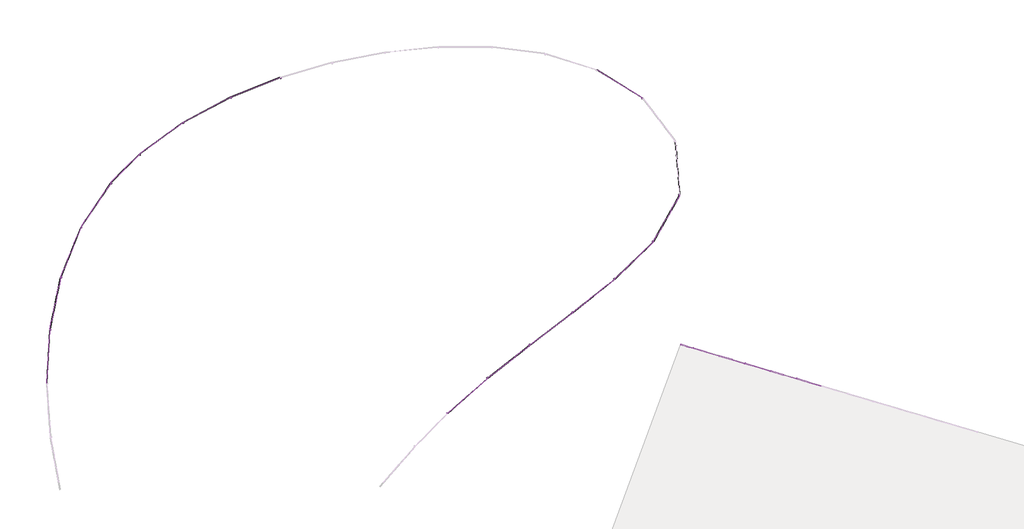
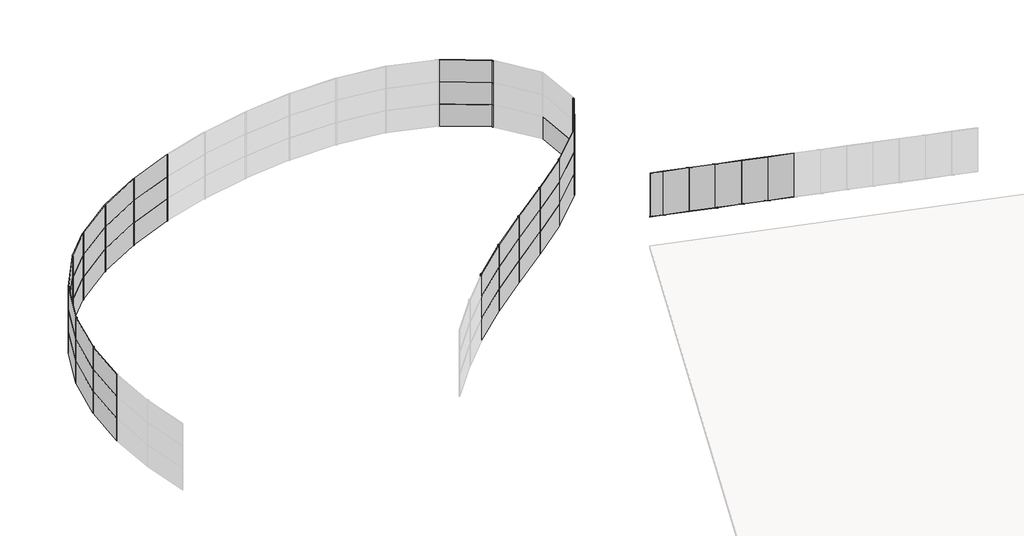
# One storey, part 4 of 5: 53 members, 52 plates.
"""IFC4 building model written with IfcOpenShell, lengths in millimetres."""

import ifcopenshell
import ifcopenshell.guid

model = None  # the IFC model being written
_history = None  # IfcOwnerHistory: only IFC2X3 demands one
_inside = {}  # id of a spatial element -> (the spatial element, [elements in it])
_under = {}  # id of a project, library or spatial element -> (it, [spatial elements below it])
_declared = {}  # id of a project -> (the project, [libraries it declares])
_typed = {}  # id of a type object -> (the type object, [elements of that type])
_made_of = {}  # id of a material, layer set ... -> (it, [elements and type objects made of it])


def new_model(schema):
    """Start an empty IFC model of exactly this schema.

    Asked for "IFC4X3", IfcOpenShell would pick the latest addendum, in which some entities
    have other attributes; the version numbers below select the first issue.
    IFC2X3 requires an IfcOwnerHistory on every rooted entity: one is made here for all.
    """
    global model, _history
    if schema == "IFC4X3":
        model = ifcopenshell.file(schema_version=(4, 3, 0, 0))
    else:
        model = ifcopenshell.file(schema=schema)
    _inside.clear()
    _under.clear()
    _declared.clear()
    _typed.clear()
    _made_of.clear()
    _history = None
    if model.schema == "IFC2X3":
        org = make("IfcOrganization", Name="unknown")
        user = make(
            "IfcPersonAndOrganization",
            ThePerson=make("IfcPerson", FamilyName="unknown"),
            TheOrganization=org,
        )
        app = make(
            "IfcApplication",
            ApplicationDeveloper=org,
            Version="unknown",
            ApplicationFullName="unknown",
            ApplicationIdentifier="unknown",
        )
        _history = make(
            "IfcOwnerHistory",
            OwningUser=user,
            OwningApplication=app,
            ChangeAction="ADDED",
            CreationDate=0,
        )
    return model


def make(cls, **values):
    """One entity of the class cls with the attributes given. An attribute that is None is left unset."""
    return model.create_entity(
        cls, **{name: value for name, value in values.items() if value is not None}
    )


def rooted(cls, **values):
    """An entity with a GlobalId (a new one), such as an element, a storey or a relation."""
    return make(cls, GlobalId=ifcopenshell.guid.new(), OwnerHistory=_history, **values)


def si_unit(unit_type, name, prefix=None):
    """IfcSIUnit, for example si_unit("LENGTHUNIT", "METRE", prefix="MILLI")."""
    return make("IfcSIUnit", UnitType=unit_type, Prefix=prefix, Name=name)


def assignment(units):
    """IfcUnitAssignment: the units of a project."""
    return None if units is None else make("IfcUnitAssignment", Units=units)


def point(xyz):
    """IfcCartesianPoint."""
    return None if xyz is None else make("IfcCartesianPoint", Coordinates=xyz)


def direction(xyz):
    """IfcDirection."""
    return None if xyz is None else make("IfcDirection", DirectionRatios=xyz)


def frame(location, z_axis=None, x_axis=None):
    """IfcAxis2Placement3D, a coordinate frame: its origin and axes. An axis left out is left unset."""
    return make(
        "IfcAxis2Placement3D",
        Location=point(location),
        Axis=direction(z_axis),
        RefDirection=direction(x_axis),
    )


def frame_2d(location, x_axis=None):
    """IfcAxis2Placement2D, a coordinate frame in the plane: its origin and x axis."""
    return make(
        "IfcAxis2Placement2D", Location=point(location), RefDirection=direction(x_axis)
    )


def origin():
    """The frame at (0, 0, 0) with its axes left unset."""
    return frame((0.0, 0.0, 0.0))


def origin_with_axes():
    """The frame at (0, 0, 0) with the z axis (0, 0, 1) and the x axis (1, 0, 0) written out."""
    return frame((0.0, 0.0, 0.0), z_axis=(0.0, 0.0, 1.0), x_axis=(1.0, 0.0, 0.0))


def origin_2d():
    """The frame at (0, 0) in the plane with its x axis left unset."""
    return frame_2d((0.0, 0.0))


def place(relative_to, where):
    """IfcLocalPlacement: puts the frame where relative to a parent placement (None: the world)."""
    return make(
        "IfcLocalPlacement", PlacementRelTo=relative_to, RelativePlacement=where
    )


def context(
    kind, dimensions, precision=None, world=None, true_north=None, identifier=None
):
    """IfcGeometricRepresentationContext, for example the 3D "Model" context."""
    return make(
        "IfcGeometricRepresentationContext",
        ContextIdentifier=identifier,
        ContextType=kind,
        CoordinateSpaceDimension=dimensions,
        Precision=precision,
        WorldCoordinateSystem=world,
        TrueNorth=true_north,
    )


def project(units=None, contexts=None):
    """IfcProject with its units and contexts."""
    return rooted(
        "IfcProject",
        Name="project",
        RepresentationContexts=contexts,
        UnitsInContext=assignment(units),
    )


def spatial(cls, under=None, at=None, **own):
    """A site, building, storey or space (cls), placed at a placement, below another one or the project."""
    s = rooted(cls, ObjectPlacement=at, **own)
    if under is not None:
        _under.setdefault(under.id(), (under, []))[1].append(s)
    return s


def polyline(points):
    """IfcPolyline through the points."""
    return make("IfcPolyline", Points=[point(p) for p in points])


def circle_curve(where, radius):
    """IfcCircle in the frame where."""
    return make("IfcCircle", Position=where, Radius=radius)


def trimmed(basis, trim1, trim2, sense, master):
    """IfcTrimmedCurve: the piece of a basis curve between two trims."""
    return make(
        "IfcTrimmedCurve",
        BasisCurve=basis,
        Trim1=trim1,
        Trim2=trim2,
        SenseAgreement=sense,
        MasterRepresentation=master,
    )


def segment(curve, same_sense, transition):
    """IfcCompositeCurveSegment."""
    return make(
        "IfcCompositeCurveSegment",
        Transition=transition,
        SameSense=same_sense,
        ParentCurve=curve,
    )


def composite_curve(segments, self_intersect=None):
    """IfcCompositeCurve: segments joined end to end."""
    return make("IfcCompositeCurve", Segments=segments, SelfIntersect=self_intersect)


def outline(outer, holes=None, kind="AREA"):
    """IfcArbitraryClosedProfileDef: a profile drawn as a closed curve; with holes, ...WithVoids."""
    if holes is None:
        return make("IfcArbitraryClosedProfileDef", ProfileType=kind, OuterCurve=outer)
    return make(
        "IfcArbitraryProfileDefWithVoids",
        ProfileType=kind,
        OuterCurve=outer,
        InnerCurves=holes,
    )


def extrude(swept, where, along, depth):
    """IfcExtrudedAreaSolid: the profile swept, set in the frame where, extruded along a direction by depth."""
    return make(
        "IfcExtrudedAreaSolid",
        SweptArea=swept,
        Position=where,
        ExtrudedDirection=direction(along),
        Depth=depth,
    )


def shape(context_of_items, identifier, shape_type, items):
    """IfcShapeRepresentation: the items that make up one representation, for example the "Body"."""
    return make(
        "IfcShapeRepresentation",
        ContextOfItems=context_of_items,
        RepresentationIdentifier=identifier,
        RepresentationType=shape_type,
        Items=items,
    )


def source(mapping_origin, context_of_items, identifier, shape_type, items):
    """IfcRepresentationMap: a shape defined once, which mapped items show again and again."""
    return make(
        "IfcRepresentationMap",
        MappingOrigin=mapping_origin,
        MappedRepresentation=shape(context_of_items, identifier, shape_type, items),
    )


def transform(
    local_origin,
    x_axis=None,
    y_axis=None,
    z_axis=None,
    scale=None,
    scale2=None,
    scale3=None,
    uniform=True,
):
    """IfcCartesianTransformationOperator3D, or its non-uniform kind. x_axis, y_axis, z_axis: its Axis1, 2, 3."""
    if uniform:
        return make(
            "IfcCartesianTransformationOperator3D",
            Axis1=direction(x_axis),
            Axis2=direction(y_axis),
            LocalOrigin=point(local_origin),
            Scale=scale,
            Axis3=direction(z_axis),
        )
    return make(
        "IfcCartesianTransformationOperator3DnonUniform",
        Axis1=direction(x_axis),
        Axis2=direction(y_axis),
        LocalOrigin=point(local_origin),
        Scale=scale,
        Axis3=direction(z_axis),
        Scale2=scale2,
        Scale3=scale3,
    )


def mapped(mapping_source, mapping_target):
    """IfcMappedItem: shows the shape of a source again, moved by a transform."""
    return make(
        "IfcMappedItem", MappingSource=mapping_source, MappingTarget=mapping_target
    )


def made_of(thing, what):
    """Note that an element or type object is made of a material, layer set ...; save() writes the relation."""
    if what is not None:
        _made_of.setdefault(what.id(), (what, []))[1].append(thing)
    return thing


def element(
    cls,
    number,
    at=None,
    inside=None,
    cuts=None,
    type_object=None,
    material=None,
    context=None,
    identifier="Body",
    shape_type=None,
    held_by="IfcProductDefinitionShape",
    body=None,
    shapes=None,
    **own,
):
    """One element of the class cls, such as IfcWall. Its Tag is "e" and its number.

    at: its placement. inside: the storey or other place that contains it. cuts: it is an
    opening in that element (IfcRelVoidsElement). A single representation is given by context,
    identifier, shape_type and body (its items); several are given by shapes. held_by: the class
    of the entity that holds the representations. save() writes the other relations.
    """
    e = rooted(cls, Tag="e%d" % number, ObjectPlacement=at, **own)
    if body is not None:
        shapes = [shape(context, identifier, shape_type, body)]
    if shapes is not None:
        e.Representation = make(held_by, Representations=shapes)
    if inside is not None:
        _inside.setdefault(inside.id(), (inside, []))[1].append(e)
    if cuts is not None:
        rooted(
            "IfcRelVoidsElement", RelatingBuildingElement=cuts, RelatedOpeningElement=e
        )
    if type_object is not None:
        _typed.setdefault(type_object.id(), (type_object, []))[1].append(e)
    return made_of(e, material)


def aggregate(whole, parts):
    """IfcRelAggregates: a whole, such as a stair, and the parts it consists of."""
    return rooted("IfcRelAggregates", RelatingObject=whole, RelatedObjects=parts)


def save(model, path):
    """Write the relations noted so far, then the file.

    IfcRelAggregates (storeys below a building ...), IfcRelContainedInSpatialStructure (elements
    in a storey), IfcRelDefinesByType, IfcRelAssociatesMaterial and IfcRelDeclares: one each for
    every whole, place, type object, material and project.
    """
    for whole, parts in _under.values():
        aggregate(whole, parts)
    for where, things in _inside.values():
        rooted(
            "IfcRelContainedInSpatialStructure",
            RelatedElements=things,
            RelatingStructure=where,
        )
    for kind, things in _typed.values():
        rooted("IfcRelDefinesByType", RelatedObjects=things, RelatingType=kind)
    for what, things in _made_of.values():
        rooted("IfcRelAssociatesMaterial", RelatedObjects=things, RelatingMaterial=what)
    for by, libraries in _declared.values():
        rooted("IfcRelDeclares", RelatingContext=by, RelatedDefinitions=libraries)
    model.write(path)


def montante_circular_25_mm_raio_36e581cf(model_context):
    return source(origin(), model_context, "Body", "SweptSolid", [
        extrude(outline(composite_curve([segment(trimmed(circle_curve(origin_2d(), 25.0), [point((25.0, 0.0))], [point((-25.0, 0.0))], False, "CARTESIAN"), True, "CONTINUOUS"), segment(trimmed(circle_curve(origin_2d(), 25.0), [point((-25.0, 0.0))], [point((25.0, 0.0))], False, "CARTESIAN"), True, "CONTINUOUS")], self_intersect=False)), frame((0.0, 0.0, -1500.0), z_axis=(0.0, 0.0, 1.0), x_axis=(1.0, 0.0, 0.0)), (0.0, 0.0, 1.0), 1500.0),
    ])


def montante_circular_25_mm_raio_a1f35a82(model_context):
    return source(origin(), model_context, "Body", "SweptSolid", [
        extrude(outline(composite_curve([segment(trimmed(circle_curve(origin_2d(), 25.0), [point((25.0, 0.0))], [point((-25.0, 0.0))], False, "CARTESIAN"), True, "CONTINUOUS"), segment(trimmed(circle_curve(origin_2d(), 25.0), [point((-25.0, 0.0))], [point((25.0, 0.0))], False, "CARTESIAN"), True, "CONTINUOUS")], self_intersect=False)), frame((0.0, 0.0, -727.4383788), z_axis=(0.0, 0.0, 1.0), x_axis=(1.0, 0.0, 0.0)), (0.0, 0.0, 1.0), 727.4383788),
    ])


def montante_circular_25_mm_raio_ce826986(model_context):
    return source(origin(), model_context, "Body", "SweptSolid", [
        extrude(outline(composite_curve([segment(trimmed(circle_curve(frame_2d((-25.0, 0.0)), 25.0), [point((0.0, 0.0))], [point((-50.0, 0.0))], False, "CARTESIAN"), True, "CONTINUOUS"), segment(trimmed(circle_curve(frame_2d((-25.0, 0.0)), 25.0), [point((-50.0, 0.0))], [point((0.0, 0.0))], False, "CARTESIAN"), True, "CONTINUOUS")], self_intersect=False)), frame((0.0, 0.0, -1500.0), z_axis=(0.0, 0.0, 1.0), x_axis=(1.0, 0.0, 0.0)), (0.0, 0.0, 1.0), 1500.0),
    ])


def painel_do_sistema_5ef9eced(model_context):
    return source(origin(), model_context, "Body", "SweptSolid", [
        extrude(outline(polyline([(1475.0, 24.5), (-1475.0, 24.5), (-1475.0, 49.5), (1475.0, 49.5), (1475.0, 24.5)])), origin_with_axes(), (0.0, 0.0, 1.0), 1500.0),
    ])


def painel_do_sistema_bf426e09(model_context):
    return source(origin(), model_context, "Body", "SweptSolid", [
        extrude(outline(polyline([(1475.0, 24.5), (-1475.0, 24.5), (-1475.0, 49.5), (1475.0, 49.5), (1475.0, 24.5)])), origin_with_axes(), (0.0, 0.0, 1.0), 727.4383788),
    ])


def painel_do_sistema_619734db(model_context):
    return source(origin(), model_context, "Body", "SweptSolid", [
        extrude(outline(polyline([(1462.5000305, -49.5), (-1462.5000305, -49.5), (-1462.5000305, -24.5), (1462.5000305, -24.5), (1462.5000305, -49.5)])), origin_with_axes(), (0.0, 0.0, 1.0), 1500.0),
    ])


def painel_do_sistema_9c2734b9(model_context):
    return source(origin(), model_context, "Body", "SweptSolid", [
        extrude(outline(polyline([(1462.5000336, -49.5), (-1462.5000336, -49.5), (-1462.5000336, -24.5), (1462.5000336, -24.5), (1462.5000336, -49.5)])), origin_with_axes(), (0.0, 0.0, 1.0), 1500.0),
    ])


def painel_do_sistema_85ccde5d(model_context):
    return source(origin(), model_context, "Body", "SweptSolid", [
        extrude(outline(polyline([(1475.0, -49.5), (-1475.0, -49.5), (-1475.0, -24.5), (1475.0, -24.5), (1475.0, -49.5)])), origin_with_axes(), (0.0, 0.0, 1.0), 1500.0),
    ])


def painel_do_sistema_91df381f(model_context):
    return source(origin(), model_context, "Body", "SweptSolid", [
        extrude(outline(polyline([(1110.3819696, -49.5), (-1110.3819696, -49.5), (-1110.3819696, -24.5), (1110.3819696, -24.5), (1110.3819696, -49.5)])), origin_with_axes(), (0.0, 0.0, 1.0), 1500.0),
    ])


model = new_model("IFC4")

# Units and contexts
model_context = context("Model", 3, world=origin())
ifc_project = project(units=[si_unit("LENGTHUNIT", "METRE", prefix="MILLI")], contexts=[model_context])

# Site, building, storey
site = spatial("IfcSite", under=ifc_project)
building = spatial("IfcBuilding", under=site)
storey = spatial("IfcBuildingStorey", under=building, Name="Nível 2", Elevation=4000.0)

# Members
placement = place(None, origin())
montante_circular_25_mm_raio_shape = montante_circular_25_mm_raio_36e581cf(model_context)
element("IfcMember", 1, ObjectType="Montante circular : 25 mm Raio", at=placement, inside=storey, context=model_context, shape_type="MappedRepresentation", body=[
    mapped(montante_circular_25_mm_raio_shape, transform((-73.9726554, 31091.8210426, 6000.000015), x_axis=(0.0, 0.0, 1.0), y_axis=(0.28318378939534855, 0.9590656606425293, 0.0), z_axis=(-0.9590656606425293, 0.28318378939534855, 0.0))),
])
element("IfcMember", 2, ObjectType="Montante circular : 25 mm Raio", at=placement, inside=storey, context=model_context, shape_type="MappedRepresentation", body=[
    mapped(montante_circular_25_mm_raio_shape, transform((-1512.5711463, 31516.5967267, 6000.000015), x_axis=(0.0, 0.0, 1.0), y_axis=(0.28318378939534644, 0.9590656606425298, 0.0), z_axis=(-0.9590656606425298, 0.28318378939534644, 0.0))),
])
element("IfcMember", 3, ObjectType="Montante circular : 25 mm Raio", at=placement, inside=storey, context=model_context, shape_type="MappedRepresentation", body=[
    mapped(montante_circular_25_mm_raio_shape, transform((-2951.1696373, 31941.3724108, 6000.000015), x_axis=(0.0, 0.0, 1.0), y_axis=(0.2831837893953519, 0.9590656606425282, 0.0), z_axis=(-0.9590656606425281, 0.2831837893953518, 0.0))),
])
element("IfcMember", 4, ObjectType="Montante circular : 25 mm Raio", at=placement, inside=storey, context=model_context, shape_type="MappedRepresentation", body=[
    mapped(montante_circular_25_mm_raio_shape, transform((-4389.7681283, 32366.1480949, 6000.000015), x_axis=(0.0, 0.0, 1.0), y_axis=(0.28318378939534594, 0.95906566064253, 0.0), z_axis=(-0.95906566064253, 0.28318378939534594, 0.0))),
])
element("IfcMember", 5, ObjectType="Montante circular : 25 mm Raio", at=placement, inside=storey, context=model_context, shape_type="MappedRepresentation", body=[
    mapped(montante_circular_25_mm_raio_shape, transform((-5828.3666192, 32790.923779, 6000.000015), x_axis=(0.0, 0.0, 1.0), y_axis=(0.283183789395347, 0.9590656606425296, 0.0), z_axis=(-0.9590656606425296, 0.283183789395347, 0.0))),
])
element("IfcMember", 6, ObjectType="Montante circular : 25 mm Raio", at=placement, inside=storey, context=model_context, shape_type="MappedRepresentation", body=[
    mapped(montante_circular_25_mm_raio_shape, transform((-40020.7762885, 39520.8946952, 4500.0), x_axis=(-0.4655884926939391, -0.8850013307735677, 0.0), y_axis=(-0.8850013307735677, 0.4655884926939391, 0.0), z_axis=(0.0, 0.0, -1.0))),
])
element("IfcMember", 7, ObjectType="Montante circular : 25 mm Raio", at=placement, inside=storey, context=model_context, shape_type="MappedRepresentation", body=[
    mapped(montante_circular_25_mm_raio_shape, transform((-41145.2595981, 36739.6113068, 4500.0), x_axis=(-0.28540905537136674, -0.958405796681147, 0.0), y_axis=(-0.958405796681147, 0.28540905537136674, 0.0), z_axis=(0.0, 0.0, -1.0))),
])
element("IfcMember", 8, ObjectType="Montante circular : 25 mm Raio", at=placement, inside=storey, context=model_context, shape_type="MappedRepresentation", body=[
    mapped(montante_circular_25_mm_raio_shape, transform((-41757.3897475, 33802.725766, 4500.0), x_axis=(-0.12631233821712995, -0.9919905207279561, 0.0), y_axis=(-0.9919905207279561, 0.12631233821712995, 0.0), z_axis=(0.0, 0.0, -1.0))),
])
element("IfcMember", 9, ObjectType="Montante circular : 25 mm Raio", at=placement, inside=storey, context=model_context, shape_type="MappedRepresentation", body=[
    mapped(montante_circular_25_mm_raio_shape, transform((-40020.7762885, 39520.8946952, 6000.0), x_axis=(-0.46558849269393926, -0.8850013307735677, 0.0), y_axis=(-0.8850013307735677, 0.46558849269393926, 0.0), z_axis=(0.0, 0.0, -1.0))),
])
element("IfcMember", 10, ObjectType="Montante circular : 25 mm Raio", at=placement, inside=storey, context=model_context, shape_type="MappedRepresentation", body=[
    mapped(montante_circular_25_mm_raio_shape, transform((-41145.2595981, 36739.6113068, 6000.0), x_axis=(-0.2854090553713671, -0.9584057966811469, 0.0), y_axis=(-0.9584057966811469, 0.2854090553713671, 0.0), z_axis=(0.0, 0.0, -1.0))),
])
element("IfcMember", 11, ObjectType="Montante circular : 25 mm Raio", at=placement, inside=storey, context=model_context, shape_type="MappedRepresentation", body=[
    mapped(montante_circular_25_mm_raio_shape, transform((-41757.3897475, 33802.725766, 6000.0), x_axis=(-0.12631233821712953, -0.9919905207279561, 0.0), y_axis=(-0.9919905207279561, 0.12631233821712953, 0.0), z_axis=(0.0, 0.0, -1.0))),
])
element("IfcMember", 12, ObjectType="Montante circular : 25 mm Raio", at=placement, inside=storey, context=model_context, shape_type="MappedRepresentation", body=[
    mapped(montante_circular_25_mm_raio_shape, transform((-40020.7762885, 39520.8946952, 7500.0), x_axis=(-0.4655884926939391, -0.8850013307735677, 0.0), y_axis=(-0.8850013307735677, 0.4655884926939391, 0.0), z_axis=(0.0, 0.0, -1.0))),
])
element("IfcMember", 13, ObjectType="Montante circular : 25 mm Raio", at=placement, inside=storey, context=model_context, shape_type="MappedRepresentation", body=[
    mapped(montante_circular_25_mm_raio_shape, transform((-41145.2595981, 36739.6113068, 7500.0), x_axis=(-0.28540905537136674, -0.958405796681147, 0.0), y_axis=(-0.958405796681147, 0.28540905537136674, 0.0), z_axis=(0.0, 0.0, -1.0))),
])
element("IfcMember", 14, ObjectType="Montante circular : 25 mm Raio", at=placement, inside=storey, context=model_context, shape_type="MappedRepresentation", body=[
    mapped(montante_circular_25_mm_raio_shape, transform((-41757.3897475, 33802.725766, 7500.0), x_axis=(-0.12631233821712995, -0.9919905207279561, 0.0), y_axis=(-0.9919905207279561, 0.12631233821712995, 0.0), z_axis=(0.0, 0.0, -1.0))),
])
element("IfcMember", 15, ObjectType="Montante circular : 25 mm Raio", at=placement, inside=storey, context=model_context, shape_type="MappedRepresentation", body=[
    mapped(montante_circular_25_mm_raio_shape, transform((-17353.3233761, 31118.8559936, 4500.0), x_axis=(0.7724767966577648, 0.6350429895883886, 0.0), y_axis=(0.6350429895883886, -0.7724767966577648, 0.0), z_axis=(0.0, 0.0, -1.0))),
])
element("IfcMember", 16, ObjectType="Montante circular : 25 mm Raio", at=placement, inside=storey, context=model_context, shape_type="MappedRepresentation", body=[
    mapped(montante_circular_25_mm_raio_shape, transform((-14996.1891623, 32974.6356945, 4500.0), x_axis=(0.7952150611070873, 0.6063274747102028, 0.0), y_axis=(0.6063274747102028, -0.7952150611070873, 0.0), z_axis=(0.0, 0.0, -1.0))),
])
element("IfcMember", 17, ObjectType="Montante circular : 25 mm Raio", at=placement, inside=storey, context=model_context, shape_type="MappedRepresentation", body=[
    mapped(montante_circular_25_mm_raio_shape, transform((-12604.1298635, 34785.1749266, 4500.0), x_axis=(0.7953870623365296, 0.6061018240095187, 0.0), y_axis=(0.6061018240095187, -0.7953870623365296, 0.0), z_axis=(0.0, 0.0, -1.0))),
])
element("IfcMember", 18, ObjectType="Montante circular : 25 mm Raio", at=placement, inside=storey, context=model_context, shape_type="MappedRepresentation", body=[
    mapped(montante_circular_25_mm_raio_shape, transform((-10255.474771, 36651.6741247, 4500.0), x_axis=(0.7627263023971693, 0.6467214142361005, 0.0), y_axis=(0.6467214142361005, -0.7627263023971693, 0.0), z_axis=(0.0, 0.0, -1.0))),
])
element("IfcMember", 19, ObjectType="Montante circular : 25 mm Raio", at=placement, inside=storey, context=model_context, shape_type="MappedRepresentation", body=[
    mapped(montante_circular_25_mm_raio_shape, transform((-8101.871437, 38740.2125323, 4500.0), x_axis=(0.6490334571140042, 0.7607598645739956, 0.0), y_axis=(0.7607598645739956, -0.6490334571140042, 0.0), z_axis=(0.0, 0.0, -1.0))),
])
element("IfcMember", 20, ObjectType="Montante circular : 25 mm Raio", at=placement, inside=storey, context=model_context, shape_type="MappedRepresentation", body=[
    mapped(montante_circular_25_mm_raio_shape, transform((-6627.5874319, 41352.9671461, 4500.0), x_axis=(0.24827563424230142, 0.9686894287859154, 0.0), y_axis=(0.9686894287859154, -0.24827563424230142, 0.0), z_axis=(0.0, 0.0, -1.0))),
])
element("IfcMember", 21, ObjectType="Montante circular : 25 mm Raio", at=placement, inside=storey, context=model_context, shape_type="MappedRepresentation", body=[
    mapped(montante_circular_25_mm_raio_shape, transform((-8685.5307871, 46730.4667655, 4500.0), x_axis=(-0.7608105002607386, 0.6489741001711892, 0.0), y_axis=(0.6489741001711892, 0.7608105002607386, 0.0), z_axis=(0.0, 0.0, -1.0))),
])
element("IfcMember", 22, ObjectType="Montante circular : 25 mm Raio", at=placement, inside=storey, context=model_context, shape_type="MappedRepresentation", body=[
    mapped(montante_circular_25_mm_raio_shape, transform((-28892.5410808, 47874.3709699, 4500.0), x_axis=(-0.9471529213375351, -0.3207823929111028, 0.0), y_axis=(-0.3207823929111028, 0.9471529213375351, 0.0), z_axis=(0.0, 0.0, -1.0))),
])
element("IfcMember", 23, ObjectType="Montante circular : 25 mm Raio", at=placement, inside=storey, context=model_context, shape_type="MappedRepresentation", body=[
    mapped(montante_circular_25_mm_raio_shape, transform((-31682.4252949, 46771.3994961, 4500.0), x_axis=(-0.9093535544571358, -0.41602417357188853, 0.0), y_axis=(-0.41602417357188853, 0.9093535544571358, 0.0), z_axis=(0.0, 0.0, -1.0))),
])
element("IfcMember", 24, ObjectType="Montante circular : 25 mm Raio", at=placement, inside=storey, context=model_context, shape_type="MappedRepresentation", body=[
    mapped(montante_circular_25_mm_raio_shape, transform((-34331.1697585, 45362.7999198, 4500.0), x_axis=(-0.850927589483555, -0.5252830070121312, 0.0), y_axis=(-0.5252830070121312, 0.850927589483555, 0.0), z_axis=(0.0, 0.0, -1.0))),
])
element("IfcMember", 25, ObjectType="Montante circular : 25 mm Raio", at=placement, inside=storey, context=model_context, shape_type="MappedRepresentation", body=[
    mapped(montante_circular_25_mm_raio_shape, transform((-36756.8303499, 43597.5320378, 4500.0), x_axis=(-0.7567414762597636, -0.6537142633507346, 0.0), y_axis=(-0.6537142633507346, 0.7567414762597636, 0.0), z_axis=(0.0, 0.0, -1.0))),
])
element("IfcMember", 26, ObjectType="Montante circular : 25 mm Raio", at=placement, inside=storey, context=model_context, shape_type="MappedRepresentation", body=[
    mapped(montante_circular_25_mm_raio_shape, transform((-17353.3233761, 31118.8559936, 6000.0), x_axis=(0.7724767966577647, 0.6350429895883888, 0.0), y_axis=(0.6350429895883888, -0.7724767966577647, 0.0), z_axis=(0.0, 0.0, -1.0))),
])
element("IfcMember", 27, ObjectType="Montante circular : 25 mm Raio", at=placement, inside=storey, context=model_context, shape_type="MappedRepresentation", body=[
    mapped(montante_circular_25_mm_raio_shape, transform((-14996.1891623, 32974.6356945, 6000.0), x_axis=(0.7952150611070872, 0.6063274747102029, 0.0), y_axis=(0.6063274747102029, -0.7952150611070872, 0.0), z_axis=(0.0, 0.0, -1.0))),
])
element("IfcMember", 28, ObjectType="Montante circular : 25 mm Raio", at=placement, inside=storey, context=model_context, shape_type="MappedRepresentation", body=[
    mapped(montante_circular_25_mm_raio_shape, transform((-12604.1298635, 34785.1749266, 6000.0), x_axis=(0.7953870623365296, 0.6061018240095187, 0.0), y_axis=(0.6061018240095187, -0.7953870623365296, 0.0), z_axis=(0.0, 0.0, -1.0))),
])
element("IfcMember", 29, ObjectType="Montante circular : 25 mm Raio", at=placement, inside=storey, context=model_context, shape_type="MappedRepresentation", body=[
    mapped(montante_circular_25_mm_raio_shape, transform((-10255.474771, 36651.6741247, 6000.0), x_axis=(0.7627263023971692, 0.6467214142361007, 0.0), y_axis=(0.6467214142361007, -0.7627263023971692, 0.0), z_axis=(0.0, 0.0, -1.0))),
])
element("IfcMember", 30, ObjectType="Montante circular : 25 mm Raio", at=placement, inside=storey, context=model_context, shape_type="MappedRepresentation", body=[
    mapped(montante_circular_25_mm_raio_shape, transform((-8101.871437, 38740.2125323, 6000.0), x_axis=(0.6490334571140043, 0.7607598645739955, 0.0), y_axis=(0.7607598645739955, -0.6490334571140043, 0.0), z_axis=(0.0, 0.0, -1.0))),
])
element("IfcMember", 31, ObjectType="Montante circular : 25 mm Raio", at=placement, inside=storey, context=model_context, shape_type="MappedRepresentation", body=[
    mapped(montante_circular_25_mm_raio_shape, transform((-6627.5874319, 41352.9671461, 6000.0), x_axis=(0.24827563424230267, 0.968689428785915, 0.0), y_axis=(0.968689428785915, -0.24827563424230267, 0.0), z_axis=(0.0, 0.0, -1.0))),
])
element("IfcMember", 32, ObjectType="Montante circular : 25 mm Raio", at=placement, inside=storey, context=model_context, shape_type="MappedRepresentation", body=[
    mapped(montante_circular_25_mm_raio_shape, transform((-8685.5307871, 46730.4667655, 6000.0), x_axis=(-0.7608105002607383, 0.6489741001711896, 0.0), y_axis=(0.6489741001711896, 0.7608105002607383, 0.0), z_axis=(0.0, 0.0, -1.0))),
])
element("IfcMember", 33, ObjectType="Montante circular : 25 mm Raio", at=placement, inside=storey, context=model_context, shape_type="MappedRepresentation", body=[
    mapped(montante_circular_25_mm_raio_shape, transform((-28892.5410808, 47874.3709699, 6000.0), x_axis=(-0.9471529213375351, -0.32078239291110255, 0.0), y_axis=(-0.32078239291110255, 0.9471529213375351, 0.0), z_axis=(0.0, 0.0, -1.0))),
])
element("IfcMember", 34, ObjectType="Montante circular : 25 mm Raio", at=placement, inside=storey, context=model_context, shape_type="MappedRepresentation", body=[
    mapped(montante_circular_25_mm_raio_shape, transform((-31682.4252949, 46771.3994961, 6000.0), x_axis=(-0.9093535544571357, -0.4160241735718888, 0.0), y_axis=(-0.4160241735718888, 0.9093535544571357, 0.0), z_axis=(0.0, 0.0, -1.0))),
])
element("IfcMember", 35, ObjectType="Montante circular : 25 mm Raio", at=placement, inside=storey, context=model_context, shape_type="MappedRepresentation", body=[
    mapped(montante_circular_25_mm_raio_shape, transform((-34331.1697585, 45362.7999198, 6000.0), x_axis=(-0.850927589483555, -0.5252830070121313, 0.0), y_axis=(-0.5252830070121313, 0.850927589483555, 0.0), z_axis=(0.0, 0.0, -1.0))),
])
element("IfcMember", 36, ObjectType="Montante circular : 25 mm Raio", at=placement, inside=storey, context=model_context, shape_type="MappedRepresentation", body=[
    mapped(montante_circular_25_mm_raio_shape, transform((-36756.8303499, 43597.5320378, 6000.0), x_axis=(-0.7567414762597636, -0.6537142633507346, 0.0), y_axis=(-0.6537142633507346, 0.7567414762597636, 0.0), z_axis=(0.0, 0.0, -1.0))),
])
element("IfcMember", 37, ObjectType="Montante circular : 25 mm Raio", at=placement, inside=storey, context=model_context, shape_type="MappedRepresentation", body=[
    mapped(montante_circular_25_mm_raio_shape, transform((-17353.3233761, 31118.8559936, 7500.0), x_axis=(0.7724767966577648, 0.6350429895883886, 0.0), y_axis=(0.6350429895883886, -0.7724767966577648, 0.0), z_axis=(0.0, 0.0, -1.0))),
])
element("IfcMember", 38, ObjectType="Montante circular : 25 mm Raio", at=placement, inside=storey, context=model_context, shape_type="MappedRepresentation", body=[
    mapped(montante_circular_25_mm_raio_shape, transform((-14996.1891623, 32974.6356945, 7500.0), x_axis=(0.7952150611070873, 0.6063274747102028, 0.0), y_axis=(0.6063274747102028, -0.7952150611070873, 0.0), z_axis=(0.0, 0.0, -1.0))),
])
element("IfcMember", 39, ObjectType="Montante circular : 25 mm Raio", at=placement, inside=storey, context=model_context, shape_type="MappedRepresentation", body=[
    mapped(montante_circular_25_mm_raio_shape, transform((-12604.1298635, 34785.1749266, 7500.0), x_axis=(0.7953870623365296, 0.6061018240095187, 0.0), y_axis=(0.6061018240095187, -0.7953870623365296, 0.0), z_axis=(0.0, 0.0, -1.0))),
])
element("IfcMember", 40, ObjectType="Montante circular : 25 mm Raio", at=placement, inside=storey, context=model_context, shape_type="MappedRepresentation", body=[
    mapped(montante_circular_25_mm_raio_shape, transform((-10255.474771, 36651.6741247, 7500.0), x_axis=(0.7627263023971693, 0.6467214142361005, 0.0), y_axis=(0.6467214142361005, -0.7627263023971693, 0.0), z_axis=(0.0, 0.0, -1.0))),
])
element("IfcMember", 41, ObjectType="Montante circular : 25 mm Raio", at=placement, inside=storey, context=model_context, shape_type="MappedRepresentation", body=[
    mapped(montante_circular_25_mm_raio_shape, transform((-8101.871437, 38740.2125323, 7500.0), x_axis=(0.6490334571140042, 0.7607598645739956, 0.0), y_axis=(0.7607598645739956, -0.6490334571140042, 0.0), z_axis=(0.0, 0.0, -1.0))),
])
element("IfcMember", 42, ObjectType="Montante circular : 25 mm Raio", at=placement, inside=storey, context=model_context, shape_type="MappedRepresentation", body=[
    mapped(montante_circular_25_mm_raio_shape, transform((-6627.5874319, 41352.9671461, 7500.0), x_axis=(0.2482756342423014, 0.9686894287859154, 0.0), y_axis=(0.9686894287859154, -0.2482756342423014, 0.0), z_axis=(0.0, 0.0, -1.0))),
])
element("IfcMember", 43, ObjectType="Montante circular : 25 mm Raio", at=placement, inside=storey, context=model_context, shape_type="MappedRepresentation", body=[
    mapped(montante_circular_25_mm_raio_shape, transform((-8685.5307871, 46730.4667655, 7500.0), x_axis=(-0.7608105002607386, 0.6489741001711892, 0.0), y_axis=(0.6489741001711892, 0.7608105002607386, 0.0), z_axis=(0.0, 0.0, -1.0))),
])
element("IfcMember", 44, ObjectType="Montante circular : 25 mm Raio", at=placement, inside=storey, context=model_context, shape_type="MappedRepresentation", body=[
    mapped(montante_circular_25_mm_raio_shape, transform((-28892.5410808, 47874.3709699, 7500.0), x_axis=(-0.9471529213375351, -0.3207823929111028, 0.0), y_axis=(-0.3207823929111028, 0.9471529213375351, 0.0), z_axis=(0.0, 0.0, -1.0))),
])
element("IfcMember", 45, ObjectType="Montante circular : 25 mm Raio", at=placement, inside=storey, context=model_context, shape_type="MappedRepresentation", body=[
    mapped(montante_circular_25_mm_raio_shape, transform((-31682.4252949, 46771.3994961, 7500.0), x_axis=(-0.9093535544571357, -0.4160241735718888, 0.0), y_axis=(-0.4160241735718888, 0.9093535544571357, 0.0), z_axis=(0.0, 0.0, -1.0))),
])
element("IfcMember", 46, ObjectType="Montante circular : 25 mm Raio", at=placement, inside=storey, context=model_context, shape_type="MappedRepresentation", body=[
    mapped(montante_circular_25_mm_raio_shape, transform((-34331.1697585, 45362.7999198, 7500.0), x_axis=(-0.8509275894835548, -0.5252830070121313, 0.0), y_axis=(-0.5252830070121313, 0.8509275894835548, 0.0), z_axis=(0.0, 0.0, -1.0))),
])
element("IfcMember", 47, ObjectType="Montante circular : 25 mm Raio", at=placement, inside=storey, context=model_context, shape_type="MappedRepresentation", body=[
    mapped(montante_circular_25_mm_raio_shape, transform((-36756.8303499, 43597.5320378, 7500.0), x_axis=(-0.7567414762597636, -0.6537142633507346, 0.0), y_axis=(-0.6537142633507346, 0.7567414762597636, 0.0), z_axis=(0.0, 0.0, -1.0))),
])
montante_circular_25_mm_raio_2_shape = montante_circular_25_mm_raio_a1f35a82(model_context)
element("IfcMember", 48, ObjectType="Montante circular : 25 mm Raio", at=placement, inside=storey, context=model_context, shape_type="MappedRepresentation", body=[
    mapped(montante_circular_25_mm_raio_2_shape, transform((-6526.0277886, 32996.9225357, 6000.000015), x_axis=(0.0, 0.0, 1.0), y_axis=(0.28318378939534294, 0.9590656606425308, 0.0), z_axis=(-0.9590656606425308, 0.28318378939534294, 0.0))),
])
montante_circular_25_mm_raio_3_shape = montante_circular_25_mm_raio_ce826986(model_context)
element("IfcMember", 49, ObjectType="Montante circular : 25 mm Raio", at=placement, inside=storey, context=model_context, shape_type="MappedRepresentation", body=[
    mapped(montante_circular_25_mm_raio_3_shape, transform((-38343.4953128, 42008.2082927, 6000.0), x_axis=(0.5590936460250615, 0.8291045139030443, 0.0), y_axis=(-0.8291045139030443, 0.5590936460250615, 0.0), z_axis=(0.0, 0.0, 1.0))),
])
element("IfcMember", 50, ObjectType="Montante circular : 25 mm Raio", at=placement, inside=storey, context=model_context, shape_type="MappedRepresentation", body=[
    mapped(montante_circular_25_mm_raio_3_shape, transform((-38343.4953128, 42008.2082927, 7500.0), x_axis=(0.5590936460250591, 0.829104513903046, 0.0), y_axis=(-0.829104513903046, 0.5590936460250591, 0.0), z_axis=(0.0, 0.0, 1.0))),
])
element("IfcMember", 51, ObjectType="Montante circular : 25 mm Raio", at=placement, inside=storey, context=model_context, shape_type="MappedRepresentation", body=[
    mapped(montante_circular_25_mm_raio_3_shape, transform((-38343.4953128, 42008.2082927, 9000.0), x_axis=(0.5590936460250591, 0.829104513903046, 0.0), y_axis=(-0.829104513903046, 0.5590936460250591, 0.0), z_axis=(0.0, 0.0, 1.0))),
])
element("IfcMember", 52, ObjectType="Montante circular : 25 mm Raio", at=placement, inside=storey, context=model_context, shape_type="MappedRepresentation", body=[
    mapped(montante_circular_25_mm_raio_3_shape, transform((-19607.9031675, 29139.747525, 7500.0), x_axis=(-0.7515265818306617, -0.6597028094543193, 0.0), y_axis=(0.6597028094543193, -0.7515265818306617, 0.0), z_axis=(0.0, 0.0, 1.0))),
])
element("IfcMember", 53, ObjectType="Montante circular : 25 mm Raio", at=placement, inside=storey, context=model_context, shape_type="MappedRepresentation", body=[
    mapped(montante_circular_25_mm_raio_3_shape, transform((-19607.9031675, 29139.747525, 9000.0), x_axis=(-0.7515265818306621, -0.6597028094543189, 0.0), y_axis=(0.6597028094543189, -0.7515265818306621, 0.0), z_axis=(0.0, 0.0, 1.0))),
])

# Plates
painel_do_sistema_shape = painel_do_sistema_5ef9eced(model_context)
element("IfcPlate", 54, ObjectType="Painel do sistema : Envidraçado", at=placement, inside=storey, context=model_context, shape_type="MappedRepresentation", body=[
    mapped(painel_do_sistema_shape, transform((-73.9726554, 31091.8210426, 7500.00001), x_axis=(0.0, 0.0, 1.0), y_axis=(-0.283183789395346, -0.95906566064253, 0.0), z_axis=(0.95906566064253, -0.283183789395346, 0.0))),
])
element("IfcPlate", 55, ObjectType="Painel do sistema : Envidraçado", at=placement, inside=storey, context=model_context, shape_type="MappedRepresentation", body=[
    mapped(painel_do_sistema_shape, transform((-1512.5711463, 31516.5967267, 7500.00001), x_axis=(0.0, 0.0, 1.0), y_axis=(-0.28318378939534916, -0.959065660642529, 0.0), z_axis=(0.959065660642529, -0.28318378939534916, 0.0))),
])
element("IfcPlate", 56, ObjectType="Painel do sistema : Envidraçado", at=placement, inside=storey, context=model_context, shape_type="MappedRepresentation", body=[
    mapped(painel_do_sistema_shape, transform((-2951.1696373, 31941.3724108, 7500.00001), x_axis=(0.0, 0.0, 1.0), y_axis=(-0.28318378939534916, -0.959065660642529, 0.0), z_axis=(0.959065660642529, -0.28318378939534916, 0.0))),
])
element("IfcPlate", 57, ObjectType="Painel do sistema : Envidraçado", at=placement, inside=storey, context=model_context, shape_type="MappedRepresentation", body=[
    mapped(painel_do_sistema_shape, transform((-4389.7681283, 32366.1480949, 7500.00001), x_axis=(0.0, 0.0, 1.0), y_axis=(-0.283183789395346, -0.95906566064253, 0.0), z_axis=(0.95906566064253, -0.283183789395346, 0.0))),
])
element("IfcPlate", 58, ObjectType="Painel do sistema : Envidraçado", at=placement, inside=storey, context=model_context, shape_type="MappedRepresentation", body=[
    mapped(painel_do_sistema_shape, transform((-5828.3666192, 32790.923779, 7500.00001), x_axis=(0.0, 0.0, 1.0), y_axis=(-0.28318378939534705, -0.9590656606425296, 0.0), z_axis=(0.9590656606425296, -0.28318378939534705, 0.0))),
])
painel_do_sistema_2_shape = painel_do_sistema_bf426e09(model_context)
element("IfcPlate", 59, ObjectType="Painel do sistema : Envidraçado", at=placement, inside=storey, context=model_context, shape_type="MappedRepresentation", body=[
    mapped(painel_do_sistema_2_shape, transform((-6526.0277886, 32996.9225357, 7500.00001), x_axis=(0.0, 0.0, 1.0), y_axis=(-0.28318378939534383, -0.9590656606425306, 0.0), z_axis=(0.9590656606425306, -0.28318378939534383, 0.0))),
])
painel_do_sistema_3_shape = painel_do_sistema_619734db(model_context)
element("IfcPlate", 60, ObjectType="Painel do sistema : Envidraçado", at=placement, inside=storey, context=model_context, shape_type="MappedRepresentation", body=[
    mapped(painel_do_sistema_3_shape, transform((-18471.2191895, 30137.5480444, 4500.0), x_axis=(0.7515265818306623, 0.6597028094543185, 0.0), y_axis=(-0.6597028094543185, 0.7515265818306623, 0.0), z_axis=(0.0, 0.0, 1.0))),
])
element("IfcPlate", 61, ObjectType="Painel do sistema : Envidraçado", at=placement, inside=storey, context=model_context, shape_type="MappedRepresentation", body=[
    mapped(painel_do_sistema_3_shape, transform((-18471.2191895, 30137.5480444, 6000.0), x_axis=(0.7515265818306617, 0.6597028094543193, 0.0), y_axis=(-0.6597028094543193, 0.7515265818306617, 0.0), z_axis=(0.0, 0.0, 1.0))),
])
element("IfcPlate", 62, ObjectType="Painel do sistema : Envidraçado", at=placement, inside=storey, context=model_context, shape_type="MappedRepresentation", body=[
    mapped(painel_do_sistema_3_shape, transform((-18471.2191895, 30137.5480444, 7500.0), x_axis=(0.7515265818306621, 0.6597028094543189, 0.0), y_axis=(-0.6597028094543189, 0.7515265818306621, 0.0), z_axis=(0.0, 0.0, 1.0))),
])
painel_do_sistema_4_shape = painel_do_sistema_9c2734b9(model_context)
element("IfcPlate", 63, ObjectType="Painel do sistema : Envidraçado", at=placement, inside=storey, context=model_context, shape_type="MappedRepresentation", body=[
    mapped(painel_do_sistema_4_shape, transform((-39189.1244712, 40754.1876875, 4500.0), x_axis=(-0.5590936460250615, -0.8291045139030443, 0.0), y_axis=(0.8291045139030443, -0.5590936460250615, 0.0), z_axis=(0.0, 0.0, 1.0))),
])
element("IfcPlate", 64, ObjectType="Painel do sistema : Envidraçado", at=placement, inside=storey, context=model_context, shape_type="MappedRepresentation", body=[
    mapped(painel_do_sistema_4_shape, transform((-39189.1244712, 40754.1876875, 6000.0), x_axis=(-0.5590936460250591, -0.829104513903046, 0.0), y_axis=(0.829104513903046, -0.5590936460250591, 0.0), z_axis=(0.0, 0.0, 1.0))),
])
element("IfcPlate", 65, ObjectType="Painel do sistema : Envidraçado", at=placement, inside=storey, context=model_context, shape_type="MappedRepresentation", body=[
    mapped(painel_do_sistema_4_shape, transform((-39189.1244712, 40754.1876875, 7500.0), x_axis=(-0.5590936460250591, -0.829104513903046, 0.0), y_axis=(0.829104513903046, -0.5590936460250591, 0.0), z_axis=(0.0, 0.0, 1.0))),
])
painel_do_sistema_5_shape = painel_do_sistema_85ccde5d(model_context)
element("IfcPlate", 66, ObjectType="Painel do sistema : Envidraçado", at=placement, inside=storey, context=model_context, shape_type="MappedRepresentation", body=[
    mapped(painel_do_sistema_5_shape, transform((-16174.7562692, 32046.745844, 4500.0), x_axis=(0.7857114046077295, 0.6185932336110289, 0.0), y_axis=(-0.6185932336110289, 0.7857114046077295, 0.0), z_axis=(0.0, 0.0, 1.0))),
])
element("IfcPlate", 67, ObjectType="Painel do sistema : Envidraçado", at=placement, inside=storey, context=model_context, shape_type="MappedRepresentation", body=[
    mapped(painel_do_sistema_5_shape, transform((-13800.1595129, 33879.9053105, 4500.0), x_axis=(0.7973530996033721, 0.6035130773669242, 0.0), y_axis=(-0.6035130773669242, 0.7973530996033721, 0.0), z_axis=(0.0, 0.0, 1.0))),
])
element("IfcPlate", 68, ObjectType="Painel do sistema : Envidraçado", at=placement, inside=storey, context=model_context, shape_type="MappedRepresentation", body=[
    mapped(painel_do_sistema_5_shape, transform((-11429.8023172, 35718.4245256, 4500.0), x_axis=(0.7828850308262363, 0.6221663993725499, 0.0), y_axis=(-0.6221663993725499, 0.7828850308262363, 0.0), z_axis=(0.0, 0.0, 1.0))),
])
element("IfcPlate", 69, ObjectType="Painel do sistema : Envidraçado", at=placement, inside=storey, context=model_context, shape_type="MappedRepresentation", body=[
    mapped(painel_do_sistema_5_shape, transform((-9178.673104, 37695.9433285, 4500.0), x_axis=(0.7178677779900108, 0.6961794691914469, 0.0), y_axis=(-0.6961794691914469, 0.7178677779900108, 0.0), z_axis=(0.0, 0.0, 1.0))),
])
element("IfcPlate", 70, ObjectType="Painel do sistema : Envidraçado", at=placement, inside=storey, context=model_context, shape_type="MappedRepresentation", body=[
    mapped(painel_do_sistema_5_shape, transform((-7364.7294344, 40046.5898392, 4500.0), x_axis=(0.49142800171697115, 0.8709182046142248, 0.0), y_axis=(-0.8709182046142248, 0.49142800171697115, 0.0), z_axis=(0.0, 0.0, 1.0))),
])
element("IfcPlate", 71, ObjectType="Painel do sistema : Envidraçado", at=placement, inside=storey, context=model_context, shape_type="MappedRepresentation", body=[
    mapped(painel_do_sistema_5_shape, transform((-6748.0851686, 42848.1194111, 4500.0), x_axis=(-0.08033182448940991, 0.9967681766460056, 0.0), y_axis=(-0.9967681766460056, -0.08033182448940991, 0.0), z_axis=(0.0, 0.0, 1.0))),
])
element("IfcPlate", 72, ObjectType="Painel do sistema : Envidraçado", at=placement, inside=storey, context=model_context, shape_type="MappedRepresentation", body=[
    mapped(painel_do_sistema_5_shape, transform((-9964.7826295, 47513.7385724, 4500.0), x_axis=(-0.8528345616365336, 0.5221812046389852, 0.0), y_axis=(-0.5221812046389852, -0.8528345616365336, 0.0), z_axis=(0.0, 0.0, 1.0))),
])
element("IfcPlate", 73, ObjectType="Painel do sistema : Envidraçado", at=placement, inside=storey, context=model_context, shape_type="MappedRepresentation", body=[
    mapped(painel_do_sistema_5_shape, transform((-30287.4831879, 47322.885233, 4500.0), x_axis=(-0.9299614046943586, -0.3676571579323536, 0.0), y_axis=(0.3676571579323536, -0.9299614046943586, 0.0), z_axis=(0.0, 0.0, 1.0))),
])
element("IfcPlate", 74, ObjectType="Painel do sistema : Envidraçado", at=placement, inside=storey, context=model_context, shape_type="MappedRepresentation", body=[
    mapped(painel_do_sistema_5_shape, transform((-33006.7975267, 46067.099708, 4500.0), x_axis=(-0.8829148212020052, -0.46953319211939787, 0.0), y_axis=(0.46953319211939787, -0.8829148212020052, 0.0), z_axis=(0.0, 0.0, 1.0))),
])
element("IfcPlate", 75, ObjectType="Painel do sistema : Envidraçado", at=placement, inside=storey, context=model_context, shape_type="MappedRepresentation", body=[
    mapped(painel_do_sistema_5_shape, transform((-35544.0000542, 44480.1659788, 4500.0), x_axis=(-0.8085535304668945, -0.5884226273432395, 0.0), y_axis=(0.5884226273432395, -0.8085535304668945, 0.0), z_axis=(0.0, 0.0, 1.0))),
])
element("IfcPlate", 76, ObjectType="Painel do sistema : Envidraçado", at=placement, inside=storey, context=model_context, shape_type="MappedRepresentation", body=[
    mapped(painel_do_sistema_5_shape, transform((-16174.7562692, 32046.745844, 6000.0), x_axis=(0.78571140460773, 0.6185932336110281, 0.0), y_axis=(-0.6185932336110281, 0.78571140460773, 0.0), z_axis=(0.0, 0.0, 1.0))),
])
element("IfcPlate", 77, ObjectType="Painel do sistema : Envidraçado", at=placement, inside=storey, context=model_context, shape_type="MappedRepresentation", body=[
    mapped(painel_do_sistema_5_shape, transform((-13800.1595129, 33879.9053105, 6000.0), x_axis=(0.7973530996033728, 0.6035130773669233, 0.0), y_axis=(-0.6035130773669233, 0.7973530996033728, 0.0), z_axis=(0.0, 0.0, 1.0))),
])
element("IfcPlate", 78, ObjectType="Painel do sistema : Envidraçado", at=placement, inside=storey, context=model_context, shape_type="MappedRepresentation", body=[
    mapped(painel_do_sistema_5_shape, transform((-11429.8023172, 35718.4245256, 6000.0), x_axis=(0.7828850308262363, 0.6221663993725499, 0.0), y_axis=(-0.6221663993725499, 0.7828850308262363, 0.0), z_axis=(0.0, 0.0, 1.0))),
])
element("IfcPlate", 79, ObjectType="Painel do sistema : Envidraçado", at=placement, inside=storey, context=model_context, shape_type="MappedRepresentation", body=[
    mapped(painel_do_sistema_5_shape, transform((-9178.673104, 37695.9433285, 6000.0), x_axis=(0.71786777799001, 0.6961794691914476, 0.0), y_axis=(-0.6961794691914476, 0.71786777799001, 0.0), z_axis=(0.0, 0.0, 1.0))),
])
element("IfcPlate", 80, ObjectType="Painel do sistema : Envidraçado", at=placement, inside=storey, context=model_context, shape_type="MappedRepresentation", body=[
    mapped(painel_do_sistema_5_shape, transform((-7364.7294344, 40046.5898392, 6000.0), x_axis=(0.49142800171697026, 0.8709182046142253, 0.0), y_axis=(-0.8709182046142253, 0.49142800171697026, 0.0), z_axis=(0.0, 0.0, 1.0))),
])
element("IfcPlate", 81, ObjectType="Painel do sistema : Envidraçado", at=placement, inside=storey, context=model_context, shape_type="MappedRepresentation", body=[
    mapped(painel_do_sistema_5_shape, transform((-9964.7826295, 47513.7385724, 6000.0), x_axis=(-0.8528345616365335, 0.5221812046389853, 0.0), y_axis=(-0.5221812046389853, -0.8528345616365335, 0.0), z_axis=(0.0, 0.0, 1.0))),
])
element("IfcPlate", 82, ObjectType="Painel do sistema : Envidraçado", at=placement, inside=storey, context=model_context, shape_type="MappedRepresentation", body=[
    mapped(painel_do_sistema_5_shape, transform((-30287.4831879, 47322.885233, 6000.0), x_axis=(-0.9299614046943586, -0.36765715793235354, 0.0), y_axis=(0.36765715793235354, -0.9299614046943586, 0.0), z_axis=(0.0, 0.0, 1.0))),
])
element("IfcPlate", 83, ObjectType="Painel do sistema : Envidraçado", at=placement, inside=storey, context=model_context, shape_type="MappedRepresentation", body=[
    mapped(painel_do_sistema_5_shape, transform((-33006.7975267, 46067.099708, 6000.0), x_axis=(-0.8829148212020058, -0.4695331921193966, 0.0), y_axis=(0.4695331921193966, -0.8829148212020058, 0.0), z_axis=(0.0, 0.0, 1.0))),
])
element("IfcPlate", 84, ObjectType="Painel do sistema : Envidraçado", at=placement, inside=storey, context=model_context, shape_type="MappedRepresentation", body=[
    mapped(painel_do_sistema_5_shape, transform((-35544.0000542, 44480.1659788, 6000.0), x_axis=(-0.8085535304668935, -0.5884226273432409, 0.0), y_axis=(0.5884226273432409, -0.8085535304668935, 0.0), z_axis=(0.0, 0.0, 1.0))),
])
element("IfcPlate", 85, ObjectType="Painel do sistema : Envidraçado", at=placement, inside=storey, context=model_context, shape_type="MappedRepresentation", body=[
    mapped(painel_do_sistema_5_shape, transform((-16174.7562692, 32046.745844, 7500.0), x_axis=(0.7857114046077298, 0.6185932336110286, 0.0), y_axis=(-0.6185932336110286, 0.7857114046077298, 0.0), z_axis=(0.0, 0.0, 1.0))),
])
element("IfcPlate", 86, ObjectType="Painel do sistema : Envidraçado", at=placement, inside=storey, context=model_context, shape_type="MappedRepresentation", body=[
    mapped(painel_do_sistema_5_shape, transform((-13800.1595129, 33879.9053105, 7500.0), x_axis=(0.7973530996033728, 0.6035130773669233, 0.0), y_axis=(-0.6035130773669233, 0.7973530996033728, 0.0), z_axis=(0.0, 0.0, 1.0))),
])
element("IfcPlate", 87, ObjectType="Painel do sistema : Envidraçado", at=placement, inside=storey, context=model_context, shape_type="MappedRepresentation", body=[
    mapped(painel_do_sistema_5_shape, transform((-11429.8023172, 35718.4245256, 7500.0), x_axis=(0.7828850308262363, 0.6221663993725499, 0.0), y_axis=(-0.6221663993725499, 0.7828850308262363, 0.0), z_axis=(0.0, 0.0, 1.0))),
])
element("IfcPlate", 88, ObjectType="Painel do sistema : Envidraçado", at=placement, inside=storey, context=model_context, shape_type="MappedRepresentation", body=[
    mapped(painel_do_sistema_5_shape, transform((-9178.673104, 37695.9433285, 7500.0), x_axis=(0.7178677779900101, 0.6961794691914476, 0.0), y_axis=(-0.6961794691914476, 0.7178677779900101, 0.0), z_axis=(0.0, 0.0, 1.0))),
])
element("IfcPlate", 89, ObjectType="Painel do sistema : Envidraçado", at=placement, inside=storey, context=model_context, shape_type="MappedRepresentation", body=[
    mapped(painel_do_sistema_5_shape, transform((-7364.7294344, 40046.5898392, 7500.0), x_axis=(0.4914280017169703, 0.8709182046142253, 0.0), y_axis=(-0.8709182046142253, 0.4914280017169703, 0.0), z_axis=(0.0, 0.0, 1.0))),
])
element("IfcPlate", 90, ObjectType="Painel do sistema : Envidraçado", at=placement, inside=storey, context=model_context, shape_type="MappedRepresentation", body=[
    mapped(painel_do_sistema_5_shape, transform((-9964.7826295, 47513.7385724, 7500.0), x_axis=(-0.8528345616365334, 0.5221812046389853, 0.0), y_axis=(-0.5221812046389853, -0.8528345616365334, 0.0), z_axis=(0.0, 0.0, 1.0))),
])
element("IfcPlate", 91, ObjectType="Painel do sistema : Envidraçado", at=placement, inside=storey, context=model_context, shape_type="MappedRepresentation", body=[
    mapped(painel_do_sistema_5_shape, transform((-30287.4831879, 47322.885233, 7500.0), x_axis=(-0.9299614046943586, -0.36765715793235354, 0.0), y_axis=(0.36765715793235354, -0.9299614046943586, 0.0), z_axis=(0.0, 0.0, 1.0))),
])
element("IfcPlate", 92, ObjectType="Painel do sistema : Envidraçado", at=placement, inside=storey, context=model_context, shape_type="MappedRepresentation", body=[
    mapped(painel_do_sistema_5_shape, transform((-33006.7975267, 46067.099708, 7500.0), x_axis=(-0.8829148212020055, -0.46953319211939726, 0.0), y_axis=(0.46953319211939726, -0.8829148212020055, 0.0), z_axis=(0.0, 0.0, 1.0))),
])
element("IfcPlate", 93, ObjectType="Painel do sistema : Envidraçado", at=placement, inside=storey, context=model_context, shape_type="MappedRepresentation", body=[
    mapped(painel_do_sistema_5_shape, transform((-35544.0000542, 44480.1659788, 7500.0), x_axis=(-0.8085535304668939, -0.5884226273432401, 0.0), y_axis=(0.5884226273432401, -0.8085535304668939, 0.0), z_axis=(0.0, 0.0, 1.0))),
])
element("IfcPlate", 94, ObjectType="Painel do sistema : Envidraçado", at=placement, inside=storey, context=model_context, shape_type="MappedRepresentation", body=[
    mapped(painel_do_sistema_5_shape, transform((-40583.0179433, 38130.253001, 4500.0), x_axis=(-0.3748277698564342, -0.9270944627946238, 0.0), y_axis=(0.9270944627946238, -0.3748277698564342, 0.0), z_axis=(0.0, 0.0, 1.0))),
])
element("IfcPlate", 95, ObjectType="Painel do sistema : Envidraçado", at=placement, inside=storey, context=model_context, shape_type="MappedRepresentation", body=[
    mapped(painel_do_sistema_5_shape, transform((-41451.3246728, 35271.1685364, 4500.0), x_axis=(-0.20404338316145404, -0.9789618469521824, 0.0), y_axis=(0.9789618469521824, -0.20404338316145404, 0.0), z_axis=(0.0, 0.0, 1.0))),
])
element("IfcPlate", 96, ObjectType="Painel do sistema : Envidraçado", at=placement, inside=storey, context=model_context, shape_type="MappedRepresentation", body=[
    mapped(painel_do_sistema_5_shape, transform((-41842.5630915, 32305.1458845, 4500.0), x_axis=(-0.05678222933342518, -0.9983865876662839, 0.0), y_axis=(0.9983865876662839, -0.05678222933342518, 0.0), z_axis=(0.0, 0.0, 1.0))),
])
element("IfcPlate", 97, ObjectType="Painel do sistema : Envidraçado", at=placement, inside=storey, context=model_context, shape_type="MappedRepresentation", body=[
    mapped(painel_do_sistema_5_shape, transform((-40583.0179433, 38130.253001, 6000.0), x_axis=(-0.3748277698564347, -0.9270944627946236, 0.0), y_axis=(0.9270944627946236, -0.3748277698564347, 0.0), z_axis=(0.0, 0.0, 1.0))),
])
element("IfcPlate", 98, ObjectType="Painel do sistema : Envidraçado", at=placement, inside=storey, context=model_context, shape_type="MappedRepresentation", body=[
    mapped(painel_do_sistema_5_shape, transform((-41451.3246728, 35271.1685364, 6000.0), x_axis=(-0.20404338316145404, -0.9789618469521824, 0.0), y_axis=(0.9789618469521824, -0.20404338316145404, 0.0), z_axis=(0.0, 0.0, 1.0))),
])
element("IfcPlate", 99, ObjectType="Painel do sistema : Envidraçado", at=placement, inside=storey, context=model_context, shape_type="MappedRepresentation", body=[
    mapped(painel_do_sistema_5_shape, transform((-41842.5630915, 32305.1458845, 6000.0), x_axis=(-0.0567822293334251, -0.9983865876662839, 0.0), y_axis=(0.9983865876662839, -0.0567822293334251, 0.0), z_axis=(0.0, 0.0, 1.0))),
])
element("IfcPlate", 100, ObjectType="Painel do sistema : Envidraçado", at=placement, inside=storey, context=model_context, shape_type="MappedRepresentation", body=[
    mapped(painel_do_sistema_5_shape, transform((-40583.0179433, 38130.253001, 7500.0), x_axis=(-0.3748277698564347, -0.9270944627946236, 0.0), y_axis=(0.9270944627946236, -0.3748277698564347, 0.0), z_axis=(0.0, 0.0, 1.0))),
])
element("IfcPlate", 101, ObjectType="Painel do sistema : Envidraçado", at=placement, inside=storey, context=model_context, shape_type="MappedRepresentation", body=[
    mapped(painel_do_sistema_5_shape, transform((-41451.3246728, 35271.1685364, 7500.0), x_axis=(-0.20404338316145404, -0.9789618469521824, 0.0), y_axis=(0.9789618469521824, -0.20404338316145404, 0.0), z_axis=(0.0, 0.0, 1.0))),
])
element("IfcPlate", 102, ObjectType="Painel do sistema : Envidraçado", at=placement, inside=storey, context=model_context, shape_type="MappedRepresentation", body=[
    mapped(painel_do_sistema_5_shape, transform((-41842.5630915, 32305.1458845, 7500.0), x_axis=(-0.056782229333425104, -0.9983865876662839, 0.0), y_axis=(0.9983865876662839, -0.056782229333425104, 0.0), z_axis=(0.0, 0.0, 1.0))),
])
painel_do_sistema_6_shape = painel_do_sistema_91df381f(model_context)
element("IfcPlate", 103, ObjectType="Painel do sistema : Envidraçado", at=placement, inside=storey, context=model_context, shape_type="MappedRepresentation", body=[
    mapped(painel_do_sistema_6_shape, transform((-37558.9942636, 42794.0239341, 4500.0), x_axis=(-0.7065145784499637, -0.7076984883675183, 0.0), y_axis=(0.7076984883675183, -0.7065145784499637, 0.0), z_axis=(0.0, 0.0, 1.0))),
])
element("IfcPlate", 104, ObjectType="Painel do sistema : Envidraçado", at=placement, inside=storey, context=model_context, shape_type="MappedRepresentation", body=[
    mapped(painel_do_sistema_6_shape, transform((-37558.9942636, 42794.0239341, 6000.0), x_axis=(-0.7065145784499646, -0.7076984883675173, 0.0), y_axis=(0.7076984883675173, -0.7065145784499646, 0.0), z_axis=(0.0, 0.0, 1.0))),
])
element("IfcPlate", 105, ObjectType="Painel do sistema : Envidraçado", at=placement, inside=storey, context=model_context, shape_type="MappedRepresentation", body=[
    mapped(painel_do_sistema_6_shape, transform((-37558.9942636, 42794.0239341, 7500.0), x_axis=(-0.7065145784499645, -0.7076984883675173, 0.0), y_axis=(0.7076984883675173, -0.7065145784499645, 0.0), z_axis=(0.0, 0.0, 1.0))),
])

save(model, "model.ifc")

# Revit data of these elements
# Type "Montante circular : 25 mm Raio"
#   built-in parameter 1007350 = 0.082021 (stored number, unit not read)
# Type "Painel do sistema : Envidraçado"
#   Construction Type Id = "GSP4R"
#   Analytic Construction = "Vidraça única Pilkington 1/8 pol"
#   Visual Light Transmittance = 0.9
#   Solar Heat Gain Coefficient = 0.86
#   Heat Transfer Coefficient (U) = 6.7069 W/(m²·K)
# Elements 1, 2, 3, 4, 5, 6, 7, 8, 9, 10, 11, 12, 13, 14, 15, 16, 17, 18, 19, 20, 21, 22, 23, 24, 25, 26, 27, 28, 29, 30, 31, 32, 33, 34, 35, 36, 37, 38, 39, 40, 41, 42, 43, 44, 45, 46, 47, 48, 49, 50, 51, 52, 53 (IfcMember, "Montante circular : 25 mm Raio")
#   Phase Created = Construção nova
#   Materials on its faces: "Alumín."
# Elements 54, 55, 56, 57, 58, 59, 60, 61, 62, 63, 64, 65, 66, 67, 68, 69, 70, 71, 72, 73, 74, 75, 76, 77, 78, 79, 80, 81, 82, 83, 84, 85, 86, 87, 88, 89, 90, 91, 92, 93, 94, 95, 96, 97, 98, 99, 100, 101, 102, 103, 104, 105 (IfcPlate, "Painel do sistema : Envidraçado")
#   Phase Created = Construção nova
#   Materials on its faces: "Vidro"
# Materials
#   "Alumín.": class "Metal", colour RGB 247 247 247, transparency 0, Description = "Alumín. 6061", Cost = 0
#   "Vidro": class "Vidro", colour RGB 0 128 192, transparency 0.9, Description = "Vidro de sílica", Cost = 0
